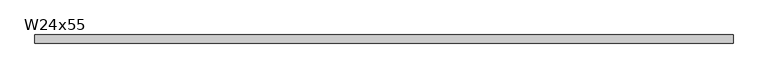
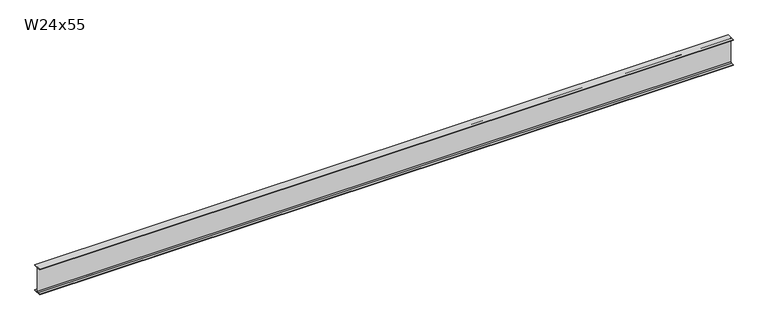
"""IFC4 building model written with IfcOpenShell, lengths in millimetres: beam geometry, RME W-Wide Flange : W24x55."""

from ifc_helpers import new_model, si_unit, point, frame, frame_2d, origin, place, context, project, spatial, polyline, circle_curve, trimmed, segment, composite_curve, outline, extrude, source, transform, mapped, element, save


def w24x55_c8ddf82d(model_context):
    return source(origin(), model_context, "Body", "SweptSolid", [
        extrude(outline(composite_curve([segment(polyline([(89.027, -286.893), (89.027, -299.72), (-89.027, -299.72), (-89.027, -286.893), (-28.702, -286.893)]), True, "CONTINUOUS"), segment(trimmed(circle_curve(frame_2d((-28.702, -263.2075)), 23.6855), [point((-28.702, -286.893))], [point((-5.0165, -263.2075))], True, "CARTESIAN"), True, "CONTINUOUS"), segment(polyline([(-5.0165, -263.2075), (-5.0165, 263.2075)]), True, "CONTINUOUS"), segment(trimmed(circle_curve(frame_2d((-28.702, 263.2075)), 23.6855), [point((-5.0165, 263.2075))], [point((-28.702, 286.893))], True, "CARTESIAN"), True, "CONTINUOUS"), segment(polyline([(-28.702, 286.893), (-89.027, 286.893), (-89.027, 299.72), (89.027, 299.72), (89.027, 286.893), (28.702, 286.893)]), True, "CONTINUOUS"), segment(trimmed(circle_curve(frame_2d((28.702, 263.2075)), 23.6855), [point((28.702, 286.893))], [point((5.0165, 263.2075))], True, "CARTESIAN"), True, "CONTINUOUS"), segment(polyline([(5.0165, 263.2075), (5.0165, -263.2075)]), True, "CONTINUOUS"), segment(trimmed(circle_curve(frame_2d((28.702, -263.2075)), 23.6855), [point((5.0165, -263.2075))], [point((28.702, -286.893))], True, "CARTESIAN"), True, "CONTINUOUS"), segment(polyline([(28.702, -286.893), (89.027, -286.893)]), True, "CONTINUOUS")], self_intersect=False)), frame((-7642.6651201, 0.0, 0.0), z_axis=(1.0, 0.0, 0.0), x_axis=(0.0, 1.0, 0.0)), (0.0, 0.0, 1.0), 15271.9973548),
    ])


if __name__ == "__main__":
    model = new_model("IFC4")
    model_context = context("Model", 3, world=origin())
    ifc_project = project(units=[si_unit("LENGTHUNIT", "METRE", prefix="MILLI")], contexts=[model_context])
    site = spatial("IfcSite", under=ifc_project)
    building = spatial("IfcBuilding", under=site)
    placement = place(None, origin())
    w24x55_shape = w24x55_c8ddf82d(model_context)
    element("IfcBeam", 1, ObjectType="RME W-Wide Flange : W24x55", at=placement, inside=building, context=model_context, shape_type="MappedRepresentation", body=[
        mapped(w24x55_shape, transform((0.0, 0.0, 0.0), x_axis=(1.0, 0.0, 0.0), y_axis=(0.0, 1.0, 0.0), z_axis=(0.0, 0.0, 1.0))),
    ])
    save(model, "model.ifc")

# Revit data of these elements
# Type "RME W-Wide Flange : W24x55"
#   WELD P [instance default] = ""
#   WELD LE [instance default] = ""
#   WELD D [instance default] = ""
#   TOP SECTION SIZE [instance default] = ""
#   TOP SECTION LENGTH [instance default] = ""
#   REMARKS [instance default] = ""
#   REINF TYPE [instance default] = ""
#   Nominal Size = "W24"
#   End Bearing Capacity [instance default] = ""
#   BOT SECTION SIZE [instance default] = ""
#   BOT SECTION LENGTH [instance default] = ""
#   Assembly Code = "B10"
#   W = 55
#   Start Extension Calculation [instance default] = 10' - 0"
#   Start Extension [instance default] = -0' - 0 1/2"
#   End Extension Calculation [instance default] = 10' - 0"
#   End Extension [instance default] = -0' - 0 1/2"
#   Length [instance default] = 5' - 0"
#   bf = 0' - 7.01"
#   d = 1' - 11.6"
#   k = 0' - 1 7/16"
#   k2 = 0' - 0.9325"
#   tf = 0' - 0.505"
#   tw = 0' - 0.395"
#   A = 0.1125 SF
#   Structural Material [instance default] = Metal - Steel - ASTM A992
# Element 1 (IfcBeam, "RME W-Wide Flange : W24x55")
#   Length = 50' - 10.25303"
#   Materials on its faces: "Metal - Steel - ASTM A992"
# Materials
#   "Metal - Steel - ASTM A992": class "Metal", colour RGB 255 128 0, transparency 0
